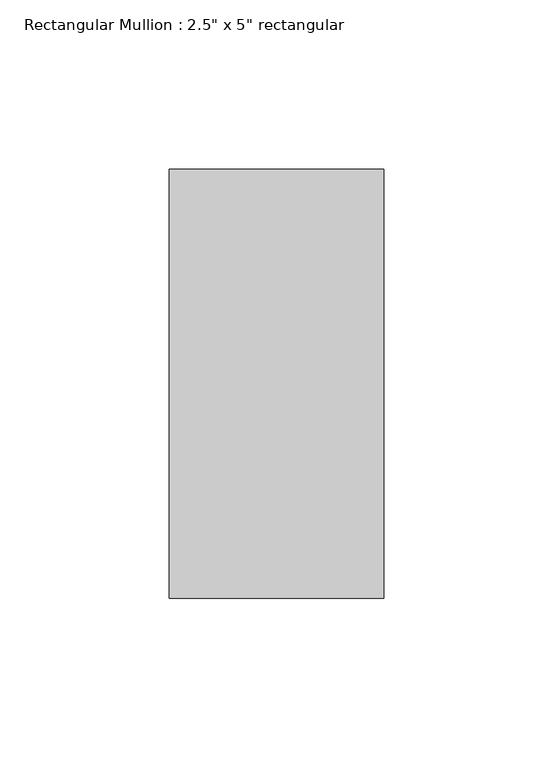
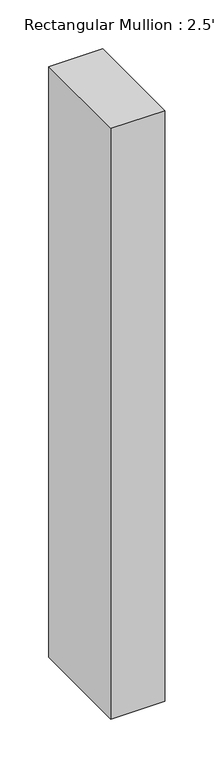
"""IFC4 building model written with IfcOpenShell, lengths in millimetres: member geometry."""

from ifc_helpers import new_model, si_unit, frame, origin, place, context, project, spatial, polyline, outline, extrude, source, transform, mapped, element, save


def member_02f00e4b(model_context):
    return source(origin(), model_context, "Body", "SweptSolid", [
        extrude(outline(polyline([(0.0, 63.5), (0.0, -63.5), (-63.5, -63.5), (-63.5, 63.5), (0.0, 63.5)])), frame((0.0, 0.0, -738.0833333), z_axis=(0.0, 0.0, 1.0), x_axis=(1.0, 0.0, 0.0)), (0.0, 0.0, 1.0), 738.0833333),
    ])


if __name__ == "__main__":
    model = new_model("IFC4")
    model_context = context("Model", 3, world=origin())
    ifc_project = project(units=[si_unit("LENGTHUNIT", "METRE", prefix="MILLI")], contexts=[model_context])
    site = spatial("IfcSite", under=ifc_project)
    building = spatial("IfcBuilding", under=site)
    placement = place(None, origin())
    member_shape = member_02f00e4b(model_context)
    element("IfcMember", 1, ObjectType="Rectangular Mullion : 2.5\" x 5\" rectangular", at=placement, inside=building, context=model_context, shape_type="MappedRepresentation", body=[
        mapped(member_shape, transform((0.0, 0.0, 0.0), x_axis=(1.0, 0.0, 0.0), y_axis=(0.0, 1.0, 0.0), z_axis=(0.0, 0.0, 1.0))),
    ])
    save(model, "model.ifc")

# Revit data of these elements
# Type "Rectangular Mullion : 2.5\" x 5\" rectangular"
#   built-in parameter 1007304 = 0.416667 (stored number, unit not read)
#   built-in parameter 1007301 = 0.104167 (stored number, unit not read)
#   built-in parameter 1007300 = 0.104167 (stored number, unit not read)
# Element 1 (IfcMember, "Rectangular Mullion : 2.5\" x 5\" rectangular")
#   Materials on its faces: "Metal - Aluminum 2"
# Materials
#   "Metal - Aluminum 2": class "Metal", colour RGB 189 187 185, transparency 0
